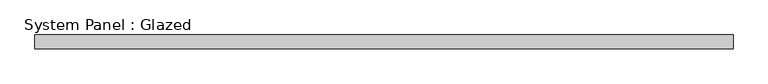
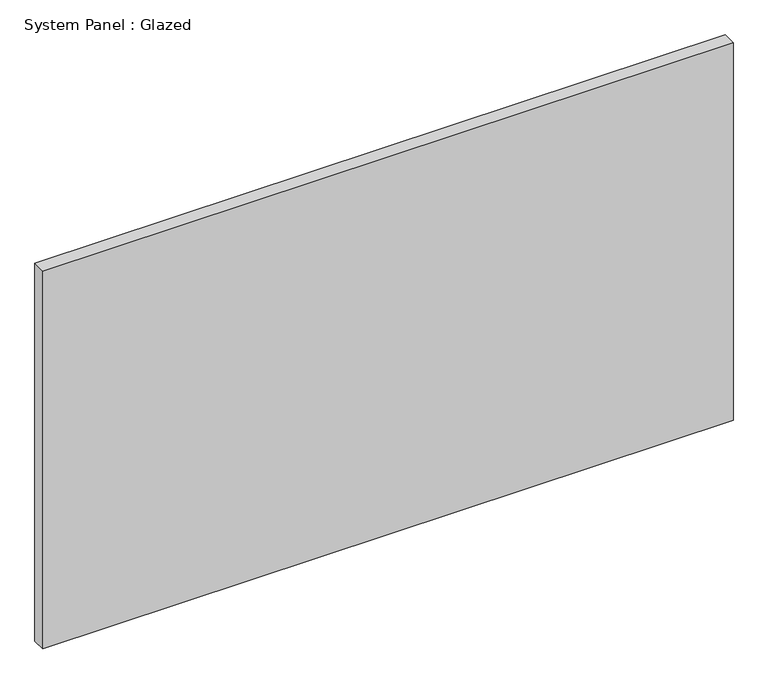
"""IFC4 building model written with IfcOpenShell, lengths in millimetres: plate geometry, System Panel : Glazed."""

import ifcopenshell
import ifcopenshell.guid

model = None  # the IFC model being written
_history = None  # IfcOwnerHistory: only IFC2X3 demands one
_inside = {}  # id of a spatial element -> (the spatial element, [elements in it])
_under = {}  # id of a project, library or spatial element -> (it, [spatial elements below it])
_declared = {}  # id of a project -> (the project, [libraries it declares])
_typed = {}  # id of a type object -> (the type object, [elements of that type])
_made_of = {}  # id of a material, layer set ... -> (it, [elements and type objects made of it])


def new_model(schema):
    """Start an empty IFC model of exactly this schema.

    Asked for "IFC4X3", IfcOpenShell would pick the latest addendum, in which some entities
    have other attributes; the version numbers below select the first issue.
    IFC2X3 requires an IfcOwnerHistory on every rooted entity: one is made here for all.
    """
    global model, _history
    if schema == "IFC4X3":
        model = ifcopenshell.file(schema_version=(4, 3, 0, 0))
    else:
        model = ifcopenshell.file(schema=schema)
    _inside.clear()
    _under.clear()
    _declared.clear()
    _typed.clear()
    _made_of.clear()
    _history = None
    if model.schema == "IFC2X3":
        org = make("IfcOrganization", Name="unknown")
        user = make(
            "IfcPersonAndOrganization",
            ThePerson=make("IfcPerson", FamilyName="unknown"),
            TheOrganization=org,
        )
        app = make(
            "IfcApplication",
            ApplicationDeveloper=org,
            Version="unknown",
            ApplicationFullName="unknown",
            ApplicationIdentifier="unknown",
        )
        _history = make(
            "IfcOwnerHistory",
            OwningUser=user,
            OwningApplication=app,
            ChangeAction="ADDED",
            CreationDate=0,
        )
    return model


def make(cls, **values):
    """One entity of the class cls with the attributes given. An attribute that is None is left unset."""
    return model.create_entity(
        cls, **{name: value for name, value in values.items() if value is not None}
    )


def rooted(cls, **values):
    """An entity with a GlobalId (a new one), such as an element, a storey or a relation."""
    return make(cls, GlobalId=ifcopenshell.guid.new(), OwnerHistory=_history, **values)


def si_unit(unit_type, name, prefix=None):
    """IfcSIUnit, for example si_unit("LENGTHUNIT", "METRE", prefix="MILLI")."""
    return make("IfcSIUnit", UnitType=unit_type, Prefix=prefix, Name=name)


def assignment(units):
    """IfcUnitAssignment: the units of a project."""
    return None if units is None else make("IfcUnitAssignment", Units=units)


def point(xyz):
    """IfcCartesianPoint."""
    return None if xyz is None else make("IfcCartesianPoint", Coordinates=xyz)


def direction(xyz):
    """IfcDirection."""
    return None if xyz is None else make("IfcDirection", DirectionRatios=xyz)


def frame(location, z_axis=None, x_axis=None):
    """IfcAxis2Placement3D, a coordinate frame: its origin and axes. An axis left out is left unset."""
    return make(
        "IfcAxis2Placement3D",
        Location=point(location),
        Axis=direction(z_axis),
        RefDirection=direction(x_axis),
    )


def origin():
    """The frame at (0, 0, 0) with its axes left unset."""
    return frame((0.0, 0.0, 0.0))


def origin_with_axes():
    """The frame at (0, 0, 0) with the z axis (0, 0, 1) and the x axis (1, 0, 0) written out."""
    return frame((0.0, 0.0, 0.0), z_axis=(0.0, 0.0, 1.0), x_axis=(1.0, 0.0, 0.0))


def place(relative_to, where):
    """IfcLocalPlacement: puts the frame where relative to a parent placement (None: the world)."""
    return make(
        "IfcLocalPlacement", PlacementRelTo=relative_to, RelativePlacement=where
    )


def context(
    kind, dimensions, precision=None, world=None, true_north=None, identifier=None
):
    """IfcGeometricRepresentationContext, for example the 3D "Model" context."""
    return make(
        "IfcGeometricRepresentationContext",
        ContextIdentifier=identifier,
        ContextType=kind,
        CoordinateSpaceDimension=dimensions,
        Precision=precision,
        WorldCoordinateSystem=world,
        TrueNorth=true_north,
    )


def project(units=None, contexts=None):
    """IfcProject with its units and contexts."""
    return rooted(
        "IfcProject",
        Name="project",
        RepresentationContexts=contexts,
        UnitsInContext=assignment(units),
    )


def spatial(cls, under=None, at=None, **own):
    """A site, building, storey or space (cls), placed at a placement, below another one or the project."""
    s = rooted(cls, ObjectPlacement=at, **own)
    if under is not None:
        _under.setdefault(under.id(), (under, []))[1].append(s)
    return s


def polyline(points):
    """IfcPolyline through the points."""
    return make("IfcPolyline", Points=[point(p) for p in points])


def outline(outer, holes=None, kind="AREA"):
    """IfcArbitraryClosedProfileDef: a profile drawn as a closed curve; with holes, ...WithVoids."""
    if holes is None:
        return make("IfcArbitraryClosedProfileDef", ProfileType=kind, OuterCurve=outer)
    return make(
        "IfcArbitraryProfileDefWithVoids",
        ProfileType=kind,
        OuterCurve=outer,
        InnerCurves=holes,
    )


def extrude(swept, where, along, depth):
    """IfcExtrudedAreaSolid: the profile swept, set in the frame where, extruded along a direction by depth."""
    return make(
        "IfcExtrudedAreaSolid",
        SweptArea=swept,
        Position=where,
        ExtrudedDirection=direction(along),
        Depth=depth,
    )


def shape(context_of_items, identifier, shape_type, items):
    """IfcShapeRepresentation: the items that make up one representation, for example the "Body"."""
    return make(
        "IfcShapeRepresentation",
        ContextOfItems=context_of_items,
        RepresentationIdentifier=identifier,
        RepresentationType=shape_type,
        Items=items,
    )


def source(mapping_origin, context_of_items, identifier, shape_type, items):
    """IfcRepresentationMap: a shape defined once, which mapped items show again and again."""
    return make(
        "IfcRepresentationMap",
        MappingOrigin=mapping_origin,
        MappedRepresentation=shape(context_of_items, identifier, shape_type, items),
    )


def transform(
    local_origin,
    x_axis=None,
    y_axis=None,
    z_axis=None,
    scale=None,
    scale2=None,
    scale3=None,
    uniform=True,
):
    """IfcCartesianTransformationOperator3D, or its non-uniform kind. x_axis, y_axis, z_axis: its Axis1, 2, 3."""
    if uniform:
        return make(
            "IfcCartesianTransformationOperator3D",
            Axis1=direction(x_axis),
            Axis2=direction(y_axis),
            LocalOrigin=point(local_origin),
            Scale=scale,
            Axis3=direction(z_axis),
        )
    return make(
        "IfcCartesianTransformationOperator3DnonUniform",
        Axis1=direction(x_axis),
        Axis2=direction(y_axis),
        LocalOrigin=point(local_origin),
        Scale=scale,
        Axis3=direction(z_axis),
        Scale2=scale2,
        Scale3=scale3,
    )


def mapped(mapping_source, mapping_target):
    """IfcMappedItem: shows the shape of a source again, moved by a transform."""
    return make(
        "IfcMappedItem", MappingSource=mapping_source, MappingTarget=mapping_target
    )


def made_of(thing, what):
    """Note that an element or type object is made of a material, layer set ...; save() writes the relation."""
    if what is not None:
        _made_of.setdefault(what.id(), (what, []))[1].append(thing)
    return thing


def element(
    cls,
    number,
    at=None,
    inside=None,
    cuts=None,
    type_object=None,
    material=None,
    context=None,
    identifier="Body",
    shape_type=None,
    held_by="IfcProductDefinitionShape",
    body=None,
    shapes=None,
    **own,
):
    """One element of the class cls, such as IfcWall. Its Tag is "e" and its number.

    at: its placement. inside: the storey or other place that contains it. cuts: it is an
    opening in that element (IfcRelVoidsElement). A single representation is given by context,
    identifier, shape_type and body (its items); several are given by shapes. held_by: the class
    of the entity that holds the representations. save() writes the other relations.
    """
    e = rooted(cls, Tag="e%d" % number, ObjectPlacement=at, **own)
    if body is not None:
        shapes = [shape(context, identifier, shape_type, body)]
    if shapes is not None:
        e.Representation = make(held_by, Representations=shapes)
    if inside is not None:
        _inside.setdefault(inside.id(), (inside, []))[1].append(e)
    if cuts is not None:
        rooted(
            "IfcRelVoidsElement", RelatingBuildingElement=cuts, RelatedOpeningElement=e
        )
    if type_object is not None:
        _typed.setdefault(type_object.id(), (type_object, []))[1].append(e)
    return made_of(e, material)


def aggregate(whole, parts):
    """IfcRelAggregates: a whole, such as a stair, and the parts it consists of."""
    return rooted("IfcRelAggregates", RelatingObject=whole, RelatedObjects=parts)


def save(model, path):
    """Write the relations noted so far, then the file.

    IfcRelAggregates (storeys below a building ...), IfcRelContainedInSpatialStructure (elements
    in a storey), IfcRelDefinesByType, IfcRelAssociatesMaterial and IfcRelDeclares: one each for
    every whole, place, type object, material and project.
    """
    for whole, parts in _under.values():
        aggregate(whole, parts)
    for where, things in _inside.values():
        rooted(
            "IfcRelContainedInSpatialStructure",
            RelatedElements=things,
            RelatingStructure=where,
        )
    for kind, things in _typed.values():
        rooted("IfcRelDefinesByType", RelatedObjects=things, RelatingType=kind)
    for what, things in _made_of.values():
        rooted("IfcRelAssociatesMaterial", RelatedObjects=things, RelatingMaterial=what)
    for by, libraries in _declared.values():
        rooted("IfcRelDeclares", RelatingContext=by, RelatedDefinitions=libraries)
    model.write(path)


def system_panel_glazed_efd17426(model_context):
    return source(origin(), model_context, "Body", "SweptSolid", [
        extrude(outline(polyline([(626.7857144, 24.5), (-626.7857144, 24.5), (-626.7857144, 49.5), (626.7857144, 49.5), (626.7857144, 24.5)])), origin_with_axes(), (0.0, 0.0, 1.0), 725.0),
    ])


if __name__ == "__main__":
    model = new_model("IFC4")
    model_context = context("Model", 3, world=origin())
    ifc_project = project(units=[si_unit("LENGTHUNIT", "METRE", prefix="MILLI")], contexts=[model_context])
    site = spatial("IfcSite", under=ifc_project)
    building = spatial("IfcBuilding", under=site)
    placement = place(None, origin())
    system_panel_glazed_shape = system_panel_glazed_efd17426(model_context)
    element("IfcPlate", 1, ObjectType="System Panel : Glazed", at=placement, inside=building, context=model_context, shape_type="MappedRepresentation", body=[
        mapped(system_panel_glazed_shape, transform((0.0, 0.0, 0.0), x_axis=(1.0, 0.0, 0.0), y_axis=(0.0, 1.0, 0.0), z_axis=(0.0, 0.0, 1.0))),
    ])
    save(model, "model.ifc")

# Revit data of these elements
# Type "System Panel : Glazed"
#   Construction Type Id = "GSP4R"
#   Analytic Construction = "1/8 in Pilkington single glazing"
#   Visual Light Transmittance = 0.9
#   Solar Heat Gain Coefficient = 0.86
#   Heat Transfer Coefficient (U) = 6.7069 W/(m²·K)
#   Define Thermal Properties by = 1
# Element 1 (IfcPlate, "System Panel : Glazed")
#   Materials on its faces: "Glass"
# Materials
#   "Glass": class "Glass", colour RGB 0 128 192, transparency 0.75, Description = "Soda Lime Glass", Cost = 0
